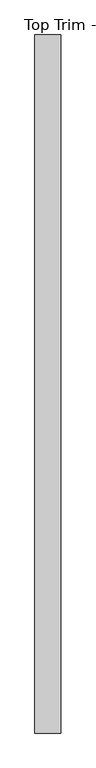
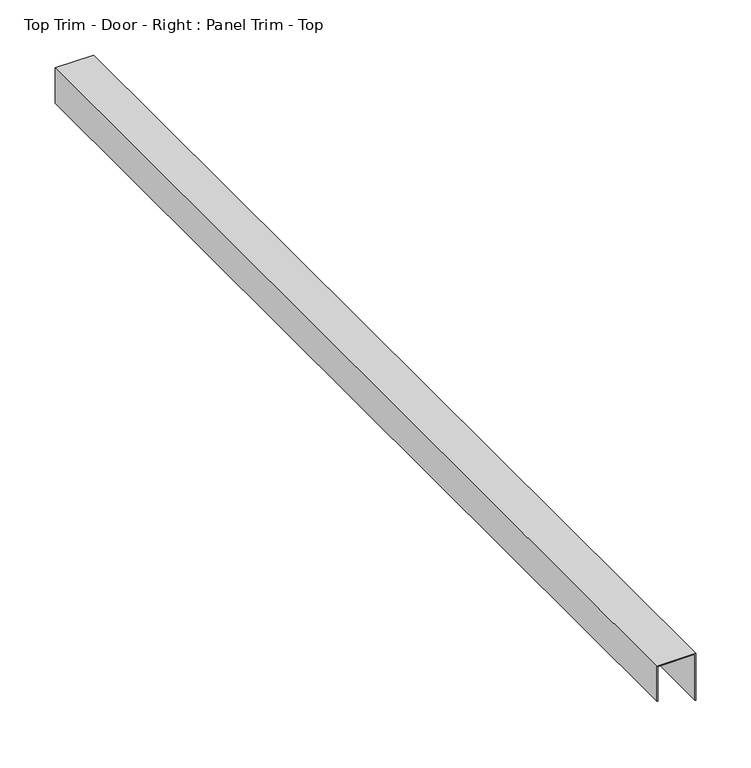
"""IFC4 building model written with IfcOpenShell, lengths in millimetres: proxy geometry, Top Trim - Door - Right : Panel Trim - Top."""

from ifc_helpers import new_model, si_unit, frame, origin, place, context, project, spatial, polyline, outline, extrude, source, transform, mapped, element, save


def top_trim_door_right_panel_trim_top_ba49df41(model_context):
    return source(origin(), model_context, "Body", "SweptSolid", [
        extrude(outline(polyline([(2438.4, 587327.0060739), (2438.4, 587365.8934739), (2387.6, 587365.8934739), (2387.6, 587366.6808739), (2439.19375, 587366.6808739), (2439.19375, 587326.2186739), (2400.3, 587326.2186739), (2400.3, 587327.0060739), (2438.4, 587327.0060739)])), frame((0.0, -533976.0163841, 0.0), z_axis=(0.0, 1.0, 0.0), x_axis=(0.0, 0.0, 1.0)), (0.0, 0.0, 1.0), 1092.2),
    ])


if __name__ == "__main__":
    model = new_model("IFC4")
    model_context = context("Model", 3, world=origin())
    ifc_project = project(units=[si_unit("LENGTHUNIT", "METRE", prefix="MILLI")], contexts=[model_context])
    site = spatial("IfcSite", under=ifc_project)
    building = spatial("IfcBuilding", under=site)
    placement = place(None, origin())
    top_trim_door_right_panel_trim_top_shape = top_trim_door_right_panel_trim_top_ba49df41(model_context)
    element("IfcBuildingElementProxy", 1, Name="Top Trim - Door - Right : Panel Trim - Top", ObjectType="Top Trim - Door - Right : Panel Trim - Top", at=placement, inside=building, context=model_context, shape_type="MappedRepresentation", body=[
        mapped(top_trim_door_right_panel_trim_top_shape, transform((0.0, 0.0, 0.0), x_axis=(1.0, 0.0, 0.0), y_axis=(0.0, 1.0, 0.0), z_axis=(0.0, 0.0, 1.0))),
    ])
    save(model, "model.ifc")

# Revit data of these elements
# Element 1 (IfcBuildingElementProxy, "Top Trim - Door - Right : Panel Trim - Top")
#   Materials on its faces: "EDGE TRIM BY MTL PANEL MFR."
# Materials
#   "EDGE TRIM BY MTL PANEL MFR.": class "Generic", colour RGB 239 242 240, transparency 0, Cost = 0
